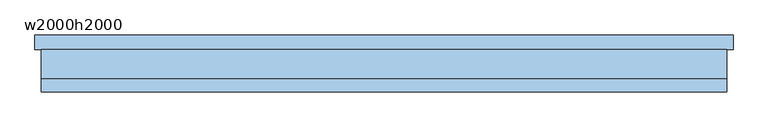
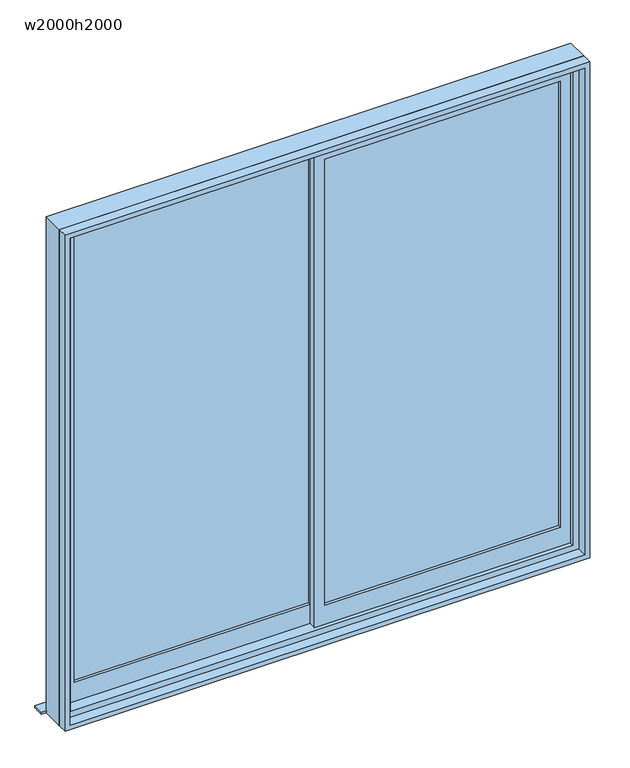
"""IFC4 building model written with IfcOpenShell, lengths in millimetres: window geometry, 引違い掃出窓_2枚 : w2000h2000."""

from ifc_helpers import new_model, si_unit, frame, origin, place, context, project, spatial, polyline, outline, extrude, source, transform, mapped, element, save


def w2000h2000_31dae58d(model_context):
    return source(origin(), model_context, "Body", "SweptSolid", [
        extrude(outline(polyline([(-20.0, 12.5), (-960.0, 12.5), (-960.0, 17.5), (-20.0, 17.5), (-20.0, 12.5)])), frame((0.0, 0.0, 80.0), z_axis=(0.0, 0.0, 1.0), x_axis=(1.0, 0.0, 0.0)), (0.0, 0.0, 1.0), 1880.0),
        extrude(outline(polyline([(960.0, -17.5), (20.0, -17.5), (20.0, -12.5), (960.0, -12.5), (960.0, -17.5)])), frame((0.0, 0.0, 80.0), z_axis=(0.0, 0.0, 1.0), x_axis=(1.0, 0.0, 0.0)), (0.0, 0.0, 1.0), 1880.0),
        extrude(outline(polyline([(2000.0, -20.0), (0.0, -20.0), (0.0, 1000.0), (2000.0, 1000.0), (2000.0, -20.0)]), holes=[polyline([(80.0, 960.0), (80.0, 20.0), (1960.0, 20.0), (1960.0, 960.0), (80.0, 960.0)])]), frame((0.0, -30.0, 0.0), z_axis=(0.0, 1.0, 0.0), x_axis=(0.0, 0.0, 1.0)), (0.0, 0.0, 1.0), 30.0),
        extrude(outline(polyline([(2000.0, -1000.0), (0.0, -1000.0), (0.0, 20.0), (2000.0, 20.0), (2000.0, -1000.0)]), holes=[polyline([(80.0, -20.0), (80.0, -960.0), (1960.0, -960.0), (1960.0, -20.0), (80.0, -20.0)])]), frame((0.0, 0.0, 0.0), z_axis=(0.0, 1.0, 0.0), x_axis=(0.0, 0.0, 1.0)), (0.0, 0.0, 1.0), 30.0),
        extrude(outline(polyline([(1065.0, 90.0), (1065.0, 45.0), (-1065.0, 45.0), (-1065.0, 90.0), (1065.0, 90.0)])), frame((0.0, 0.0, -45.0), z_axis=(0.0, 0.0, 1.0), x_axis=(1.0, 0.0, 0.0)), (0.0, 0.0, 1.0), 10.0),
        extrude(outline(polyline([(2045.0, 1045.0), (2045.0, -1045.0), (-45.0, -1045.0), (-45.0, 1045.0), (2045.0, 1045.0)]), holes=[polyline([(-25.0, -1025.0), (2025.0, -1025.0), (2025.0, 1025.0), (-25.0, 1025.0), (-25.0, -1025.0)])]), frame((0.0, -85.0, 0.0), z_axis=(0.0, 1.0, 0.0), x_axis=(0.0, 0.0, 1.0)), (0.0, 0.0, 1.0), 40.0),
        extrude(outline(polyline([(2045.0, -1045.0), (-45.0, -1045.0), (-45.0, 1045.0), (2045.0, 1045.0), (2045.0, -1045.0)]), holes=[polyline([(2000.0, 1000.0), (0.0, 1000.0), (0.0, -1000.0), (2000.0, -1000.0), (2000.0, 1000.0)])]), frame((0.0, -45.0, 0.0), z_axis=(0.0, 1.0, 0.0), x_axis=(0.0, 0.0, 1.0)), (0.0, 0.0, 1.0), 90.0),
    ])


if __name__ == "__main__":
    model = new_model("IFC4")
    model_context = context("Model", 3, world=origin())
    ifc_project = project(units=[si_unit("LENGTHUNIT", "METRE", prefix="MILLI")], contexts=[model_context])
    site = spatial("IfcSite", under=ifc_project)
    building = spatial("IfcBuilding", under=site)
    placement = place(None, origin())
    w2000h2000_shape = w2000h2000_31dae58d(model_context)
    element("IfcWindow", 1, ObjectType="引違い掃出窓_2枚 : w2000h2000", at=placement, inside=building, context=model_context, shape_type="MappedRepresentation", body=[
        mapped(w2000h2000_shape, transform((0.0, 0.0, 0.0), x_axis=(1.0, 0.0, 0.0), y_axis=(0.0, 1.0, 0.0), z_axis=(0.0, 0.0, 1.0))),
    ])
    save(model, "model.ifc")

# Revit data of these elements
# Type "引違い掃出窓_2枚 : w2000h2000"
#   Construction Type Id = "GSP4R"
#   Analytic Construction = "1/8 インチ ピルキントン一重ガラス"
#   Type Mark = "70"
#   Operation = "ダブル パネル縦"
#   Keynote = "08520.R1"
#   Visual Light Transmittance = 0.9
#   Solar Heat Gain Coefficient = 0.86
#   Heat Transfer Coefficient (U) = 6.7069 W/(m²·K)
#   Height = 2000 mm
#   既定の腰高 = 0 mm
#   Width = 2000 mm
#   額縁見附 = 20 mm
#   額縁ちり = 10 mm
#   サッシ見附 = 45 mm
#   サッシの幅 = 90 mm
#   サッシ額縁 [instance default] = none
#   サッシ本体 [instance default] = none
#   サッシガラス [instance default] = ガラス - 透明
#   Manufacturer = ""
#   Wall Closure = (empty or 0)
#   Model = ""
#   Type Comments = ""
#   Assembly Code = ""
# Element 1 (IfcWindow, "引違い掃出窓_2枚 : w2000h2000")
#   Materials on its faces: "ガラス - 透明"
# Materials
#   "ガラス - 透明": class "ガラス", colour RGB 0 128 192, transparency 0.9, Cost = 0
